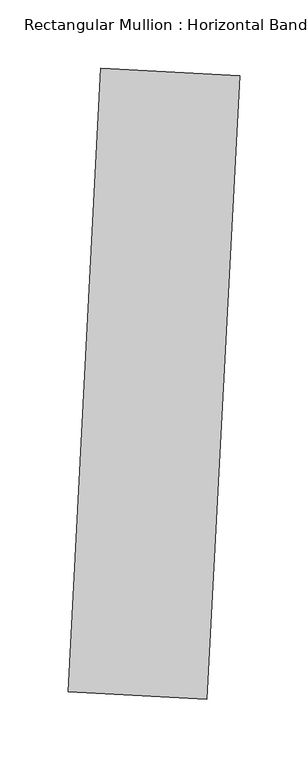
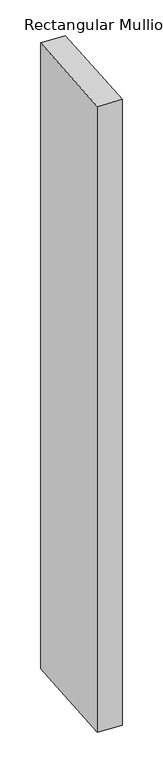
"""IFC4 building model written with IfcOpenShell, lengths in millimetres: member geometry, Rectangular Mullion : Horizontal Band."""

from ifc_helpers import new_model, si_unit, frame, origin, place, context, project, spatial, polyline, outline, extrude, source, transform, mapped, element, save


def rectangular_mullion_horizontal_band_d2a936e7(model_context):
    return source(origin(), model_context, "Body", "SweptSolid", [
        extrude(outline(polyline([(62.69438, 301.8280451), (38.7663808, -154.7453782), (-62.69438, -149.4280451), (-38.7663808, 307.1453782), (62.69438, 301.8280451)])), frame((0.0, 0.0, -2795.383136), z_axis=(0.0, 0.0, 1.0), x_axis=(1.0, 0.0, 0.0)), (0.0, 0.0, 1.0), 2795.383136),
    ])


if __name__ == "__main__":
    model = new_model("IFC4")
    model_context = context("Model", 3, world=origin())
    ifc_project = project(units=[si_unit("LENGTHUNIT", "METRE", prefix="MILLI")], contexts=[model_context])
    site = spatial("IfcSite", under=ifc_project)
    building = spatial("IfcBuilding", under=site)
    placement = place(None, origin())
    rectangular_mullion_horizontal_band_shape = rectangular_mullion_horizontal_band_d2a936e7(model_context)
    element("IfcMember", 1, ObjectType="Rectangular Mullion : Horizontal Band", at=placement, inside=building, context=model_context, shape_type="MappedRepresentation", body=[
        mapped(rectangular_mullion_horizontal_band_shape, transform((0.0, 0.0, 0.0), x_axis=(1.0, 0.0, 0.0), y_axis=(0.0, 1.0, 0.0), z_axis=(0.0, 0.0, 1.0))),
    ])
    save(model, "model.ifc")

# Revit data of these elements
# Type "Rectangular Mullion : Horizontal Band"
#   built-in parameter 1007351 = 0.25 (stored number, unit not read)
#   built-in parameter 1007304 = 1.5 (stored number, unit not read)
#   built-in parameter 1007301 = 0.166667 (stored number, unit not read)
#   built-in parameter 1007300 = 0.166667 (stored number, unit not read)
# Element 1 (IfcMember, "Rectangular Mullion : Horizontal Band")
#   Materials on its faces: "Aluminum"
# Materials
#   "Aluminum": class "Metal", colour RGB 247 247 247, transparency 0, Description = "Aluminum 6061", Cost = 0
